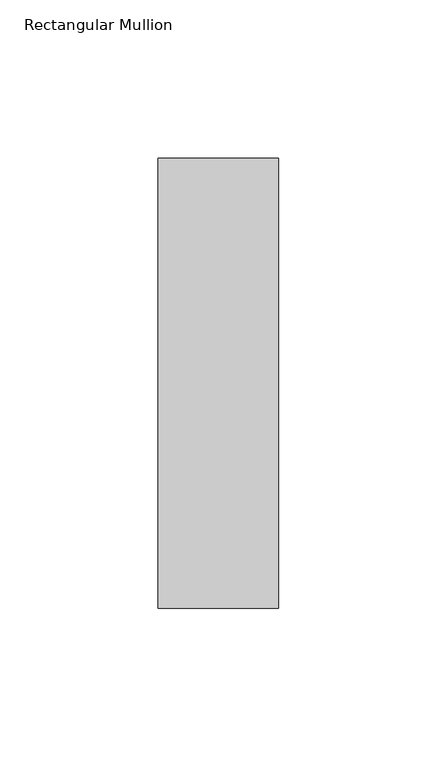
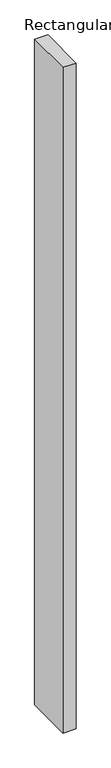
"""IFC4 building model written with IfcOpenShell, lengths in millimetres: member geometry, Rectangular Mullion : NLRS_21_CWM_hsb-regel 38x142_gen_rsf."""

from ifc_helpers import new_model, si_unit, frame, origin, place, context, project, spatial, polyline, outline, extrude, source, transform, mapped, element, save


def rectangular_mullion_39366410(model_context):
    return source(origin(), model_context, "Body", "SweptSolid", [
        extrude(outline(polyline([(19.0, -71.0), (-19.0, -71.0), (-19.0, 71.0), (19.0, 71.0), (19.0, -71.0)])), frame((0.0, 0.0, -2038.0), z_axis=(0.0, 0.0, 1.0), x_axis=(1.0, 0.0, 0.0)), (0.0, 0.0, 1.0), 2038.0),
    ])


if __name__ == "__main__":
    model = new_model("IFC4")
    model_context = context("Model", 3, world=origin())
    ifc_project = project(units=[si_unit("LENGTHUNIT", "METRE", prefix="MILLI")], contexts=[model_context])
    site = spatial("IfcSite", under=ifc_project)
    building = spatial("IfcBuilding", under=site)
    placement = place(None, origin())
    rectangular_mullion_shape = rectangular_mullion_39366410(model_context)
    element("IfcMember", 1, ObjectType="Rectangular Mullion : NLRS_21_CWM_hsb-regel 38x142_gen_rsf", at=placement, inside=building, context=model_context, shape_type="MappedRepresentation", body=[
        mapped(rectangular_mullion_shape, transform((0.0, 0.0, 0.0), x_axis=(1.0, 0.0, 0.0), y_axis=(0.0, 1.0, 0.0), z_axis=(0.0, 0.0, 1.0))),
    ])
    save(model, "model.ifc")

# Revit data of these elements
# Type "Rectangular Mullion : NLRS_21_CWM_hsb-regel 38x142_gen_rsf"
#   Export Type to IFC As = "IfcWall"
#   Type IfcGUID = "07M7mRoiH1CR8m_RSKIwpF"
#   Assembly Code = "21.10"
#   built-in parameter 1007322 = 0.465879 (stored number, unit not read)
#   built-in parameter 1007321 = 0.062336 (stored number, unit not read)
#   built-in parameter 1007320 = 0.062336 (stored number, unit not read)
# Element 1 (IfcMember, "Rectangular Mullion : NLRS_21_CWM_hsb-regel 38x142_gen_rsf")
#   Materials on its faces: "NLRS_i2_hout naaldhout vuren_gen_rsf"
# Materials
#   "NLRS_i2_hout naaldhout vuren_gen_rsf": class "I - Hout", colour RGB 234 199 147, transparency 0, Keynote = "i2", Manufacturer = "Revit Standards Foundation", URL = "www.revitstandards.org", Description = "hout vuren", Cost = 0
